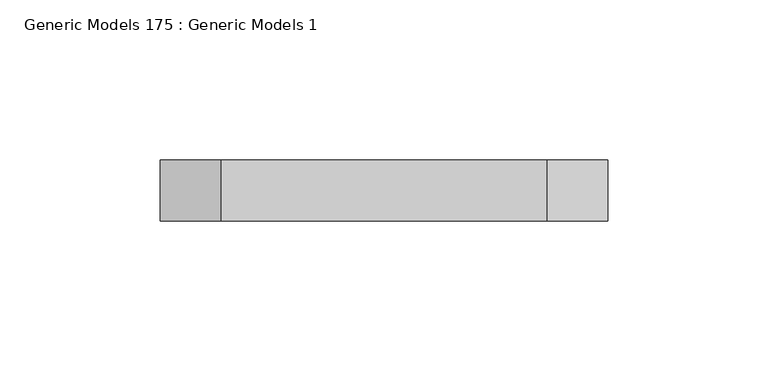
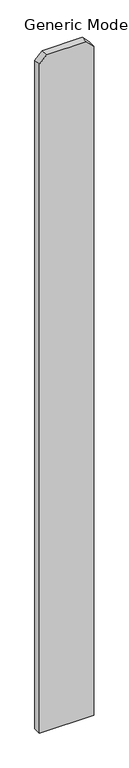
"""IFC4 building model written with IfcOpenShell, lengths in millimetres: proxy geometry, Generic Models 175 : Generic Models 1."""

from ifc_helpers import new_model, si_unit, frame, origin, place, context, project, spatial, polyline, outline, extrude, source, transform, mapped, element, save


def generic_models_175_generic_models_1_782693d9(model_context):
    return source(origin(), model_context, "Body", "SweptSolid", [
        extrude(outline(polyline([(76.2, 56665.8125), (1885.95, 56665.8125), (1905.0, 56646.7625), (1905.0, 56545.1625), (1885.95, 56526.1125), (76.2, 56526.1125), (76.2, 56665.8125)])), frame((0.0, 547.6875, 0.0), z_axis=(0.0, 1.0, 0.0), x_axis=(0.0, 0.0, 1.0)), (0.0, 0.0, 1.0), 19.05),
    ])


if __name__ == "__main__":
    model = new_model("IFC4")
    model_context = context("Model", 3, world=origin())
    ifc_project = project(units=[si_unit("LENGTHUNIT", "METRE", prefix="MILLI")], contexts=[model_context])
    site = spatial("IfcSite", under=ifc_project)
    building = spatial("IfcBuilding", under=site)
    placement = place(None, origin())
    generic_models_175_generic_models_1_shape = generic_models_175_generic_models_1_782693d9(model_context)
    element("IfcBuildingElementProxy", 1, Name="Generic Models 175 : Generic Models 1", ObjectType="Generic Models 175 : Generic Models 1", at=placement, inside=building, context=model_context, shape_type="MappedRepresentation", body=[
        mapped(generic_models_175_generic_models_1_shape, transform((0.0, 0.0, 0.0), x_axis=(1.0, 0.0, 0.0), y_axis=(0.0, 1.0, 0.0), z_axis=(0.0, 0.0, 1.0))),
    ])
    save(model, "model.ifc")

# Revit data of these elements
# Element 1 (IfcBuildingElementProxy, "Generic Models 175 : Generic Models 1")
#   Materials on its faces: "VERTICAL 1X6 CEDAR PLANKS W/ CLEAR WOOD SEALER"
# Materials
#   "VERTICAL 1X6 CEDAR PLANKS W/ CLEAR WOOD SEALER": class "Wood", colour RGB 234 198 147, transparency 0, Description = "Pinus Echinata", Cost = 0
